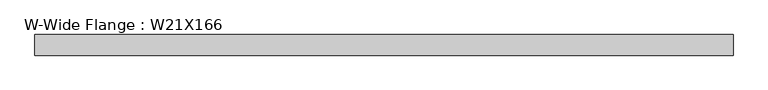
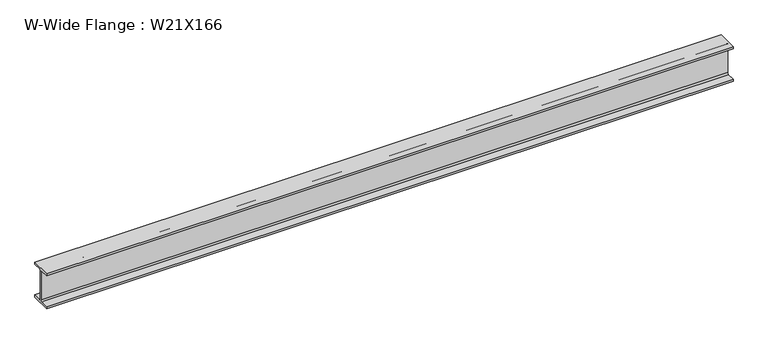
"""IFC4 building model written with IfcOpenShell, lengths in millimetres: beam geometry, W-Wide Flange : W21X166."""

from ifc_helpers import new_model, si_unit, point, frame, frame_2d, origin, place, context, project, spatial, polyline, circle_curve, trimmed, segment, composite_curve, outline, extrude, source, transform, mapped, element, save


def w_wide_flange_w21x166_a36ef0f2(model_context):
    return source(origin(), model_context, "Body", "SweptSolid", [
        extrude(outline(composite_curve([segment(polyline([(157.48, -251.206), (157.48, -285.75), (-157.48, -285.75), (-157.48, -251.206), (-32.131, -251.206)]), True, "CONTINUOUS"), segment(trimmed(circle_curve(frame_2d((-32.131, -228.6)), 22.606), [point((-32.131, -251.206))], [point((-9.525, -228.6))], True, "CARTESIAN"), True, "CONTINUOUS"), segment(polyline([(-9.525, -228.6), (-9.525, 228.6)]), True, "CONTINUOUS"), segment(trimmed(circle_curve(frame_2d((-32.131, 228.6)), 22.606), [point((-9.525, 228.6))], [point((-32.131, 251.206))], True, "CARTESIAN"), True, "CONTINUOUS"), segment(polyline([(-32.131, 251.206), (-157.48, 251.206), (-157.48, 285.75), (157.48, 285.75), (157.48, 251.206), (32.131, 251.206)]), True, "CONTINUOUS"), segment(trimmed(circle_curve(frame_2d((32.131, 228.6)), 22.606), [point((32.131, 251.206))], [point((9.525, 228.6))], True, "CARTESIAN"), True, "CONTINUOUS"), segment(polyline([(9.525, 228.6), (9.525, -228.6)]), True, "CONTINUOUS"), segment(trimmed(circle_curve(frame_2d((32.131, -228.6)), 22.606), [point((9.525, -228.6))], [point((32.131, -251.206))], True, "CARTESIAN"), True, "CONTINUOUS"), segment(polyline([(32.131, -251.206), (157.48, -251.206)]), True, "CONTINUOUS")], self_intersect=False)), frame((-5432.3588829, 0.0, 0.0), z_axis=(1.0, 0.0, 0.0), x_axis=(0.0, 1.0, 0.0)), (0.0, 0.0, 1.0), 10659.8214497),
    ])


if __name__ == "__main__":
    model = new_model("IFC4")
    model_context = context("Model", 3, world=origin())
    ifc_project = project(units=[si_unit("LENGTHUNIT", "METRE", prefix="MILLI")], contexts=[model_context])
    site = spatial("IfcSite", under=ifc_project)
    building = spatial("IfcBuilding", under=site)
    placement = place(None, origin())
    w_wide_flange_w21x166_shape = w_wide_flange_w21x166_a36ef0f2(model_context)
    element("IfcBeam", 1, ObjectType="W-Wide Flange : W21X166", at=placement, inside=building, context=model_context, shape_type="MappedRepresentation", body=[
        mapped(w_wide_flange_w21x166_shape, transform((0.0, 0.0, 0.0), x_axis=(1.0, 0.0, 0.0), y_axis=(0.0, 1.0, 0.0), z_axis=(0.0, 0.0, 1.0))),
    ])
    save(model, "model.ifc")

# Revit data of these elements
# Type "W-Wide Flange : W21X166"
#   Assembly Code = "B10"
#   W = 166
#   Length [instance default] = 5' - 0"
#   bf = 1' - 0.4"
#   d = 1' - 10 1/2"
#   k = 0' - 2 1/4"
#   k2 = 0' - 0.89"
#   tf = 0' - 1.36"
#   tw = 0' - 0 3/4"
#   A = 0.338889 SF
#   Structural Material [instance default] = Steel ASTM A992
# Element 1 (IfcBeam, "W-Wide Flange : W21X166")
#   Structural Material = Steel
#   Materials on its faces: "Steel"
# Materials
#   "Steel ASTM A992": class "Metal", colour RGB 199 199 199, transparency 0, Description = "Structural steel 50ksi", Cost = 0
#   "Steel": class "Metal", colour RGB 118 118 114, transparency 0, Description = "Steel, mill finish", Cost = 0
